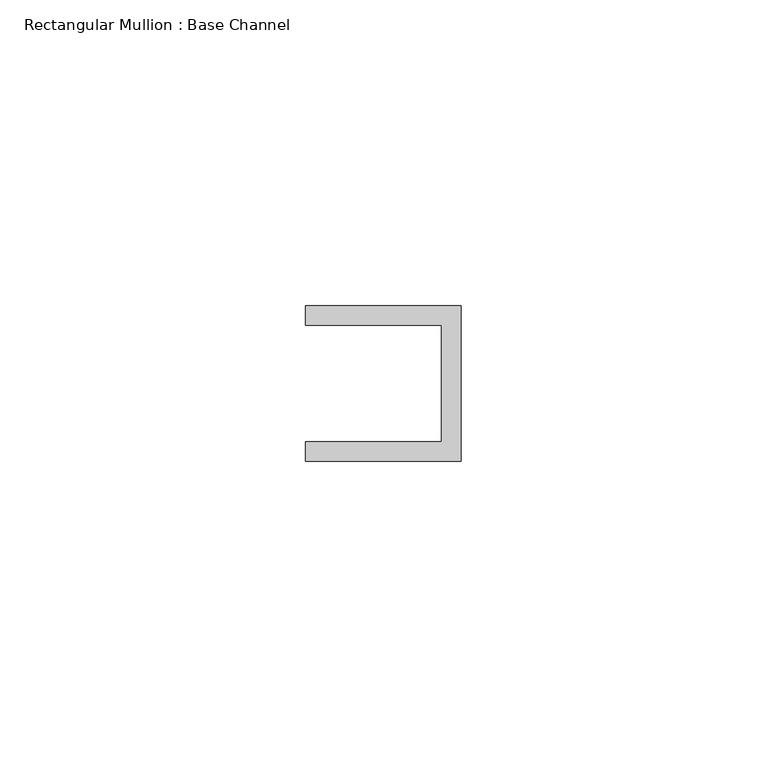
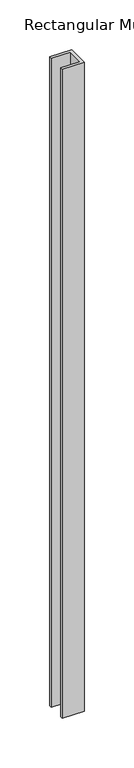
"""IFC4 building model written with IfcOpenShell, lengths in millimetres: member geometry, Rectangular Mullion : Base Channel."""

from ifc_helpers import new_model, si_unit, frame, origin, place, context, project, spatial, polyline, outline, extrude, source, transform, mapped, element, save


def rectangular_mullion_base_channel_bb8e3c89(model_context):
    return source(origin(), model_context, "Body", "SweptSolid", [
        extrude(outline(polyline([(0.0, -12.7), (-25.4, -12.7), (-25.4, -9.525), (-3.175, -9.525), (-3.175, 9.525), (-25.4, 9.525), (-25.4, 12.7), (0.0, 12.7), (0.0, -12.7)])), frame((0.0, 0.0, -797.4591001), z_axis=(0.0, 0.0, 1.0), x_axis=(1.0, 0.0, 0.0)), (0.0, 0.0, 1.0), 797.4591001),
    ])


if __name__ == "__main__":
    model = new_model("IFC4")
    model_context = context("Model", 3, world=origin())
    ifc_project = project(units=[si_unit("LENGTHUNIT", "METRE", prefix="MILLI")], contexts=[model_context])
    site = spatial("IfcSite", under=ifc_project)
    building = spatial("IfcBuilding", under=site)
    placement = place(None, origin())
    rectangular_mullion_base_channel_shape = rectangular_mullion_base_channel_bb8e3c89(model_context)
    element("IfcMember", 1, ObjectType="Rectangular Mullion : Base Channel", at=placement, inside=building, context=model_context, shape_type="MappedRepresentation", body=[
        mapped(rectangular_mullion_base_channel_shape, transform((0.0, 0.0, 0.0), x_axis=(1.0, 0.0, 0.0), y_axis=(0.0, 1.0, 0.0), z_axis=(0.0, 0.0, 1.0))),
    ])
    save(model, "model.ifc")

# Revit data of these elements
# Type "Rectangular Mullion : Base Channel"
#   built-in parameter 1007322 = 0.0833333 (stored number, unit not read)
#   built-in parameter 1007321 = 0.0416667 (stored number, unit not read)
#   built-in parameter 1007320 = -0.03125 (stored number, unit not read)
# Element 1 (IfcMember, "Rectangular Mullion : Base Channel")
#   Materials on its faces: "ALUM"
# Materials
#   "ALUM": class "Generic", colour RGB 157 157 157, transparency 0, Cost = 0
